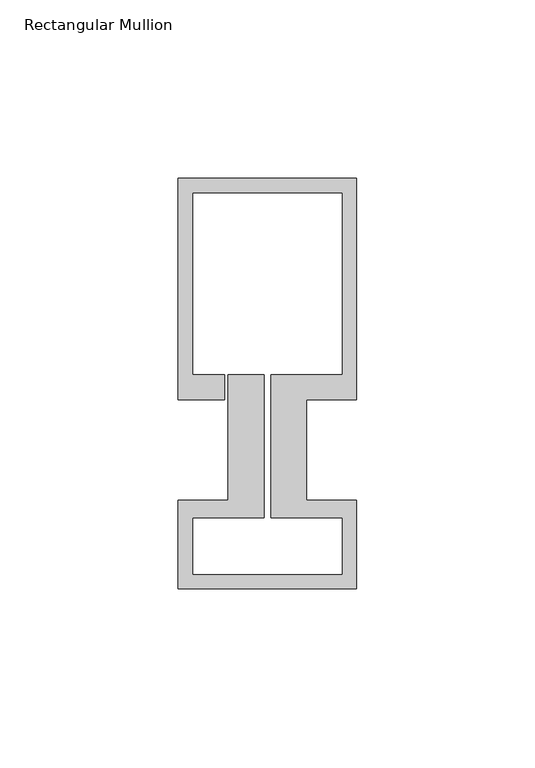
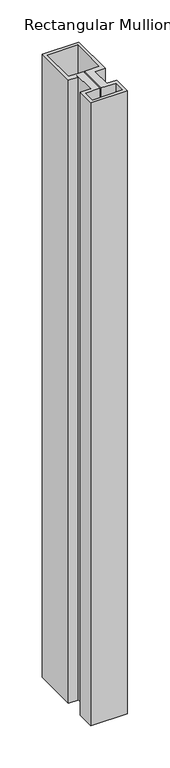
"""IFC4 building model written with IfcOpenShell, lengths in millimetres: member geometry, Rectangular Mullion : Schueco_FWS-50-HI_Tran_CovCap-20mm_Tran-55mm."""

from ifc_helpers import new_model, si_unit, frame, origin, place, context, project, spatial, polyline, outline, extrude, source, transform, mapped, element, save


def rectangular_mullion_16556d00(model_context):
    return source(origin(), model_context, "Body", "SweptSolid", [
        extrude(outline(polyline([(0.0, 90.0), (0.0, 28.0), (-14.0, 28.0), (-14.0, -0.1), (0.0, -0.1), (0.0, -25.0), (-50.0, -25.0), (-50.0, -0.1), (-36.0, -0.1), (-36.0, 35.0), (-26.0, 35.0), (-26.0, -5.0), (-46.0, -5.0), (-46.0, -21.0), (-4.0, -21.0), (-4.0, -5.0), (-24.0, -5.0), (-24.0, 35.0), (-4.0, 35.0), (-4.0, 86.0), (-46.0, 86.0), (-46.0, 35.0), (-37.0, 35.0), (-37.0, 28.0), (-50.0, 28.0), (-50.0, 90.0), (0.0, 90.0)])), frame((0.0, 0.0, -900.0), z_axis=(0.0, 0.0, 1.0), x_axis=(1.0, 0.0, 0.0)), (0.0, 0.0, 1.0), 900.0),
    ])


if __name__ == "__main__":
    model = new_model("IFC4")
    model_context = context("Model", 3, world=origin())
    ifc_project = project(units=[si_unit("LENGTHUNIT", "METRE", prefix="MILLI")], contexts=[model_context])
    site = spatial("IfcSite", under=ifc_project)
    building = spatial("IfcBuilding", under=site)
    placement = place(None, origin())
    rectangular_mullion_shape = rectangular_mullion_16556d00(model_context)
    element("IfcMember", 1, ObjectType="Rectangular Mullion : Schueco_FWS-50-HI_Tran_CovCap-20mm_Tran-55mm", at=placement, inside=building, context=model_context, shape_type="MappedRepresentation", body=[
        mapped(rectangular_mullion_shape, transform((0.0, 0.0, 0.0), x_axis=(1.0, 0.0, 0.0), y_axis=(0.0, 1.0, 0.0), z_axis=(0.0, 0.0, 1.0))),
    ])
    save(model, "model.ifc")

# Revit data of these elements
# Type "Rectangular Mullion : Schueco_FWS-50-HI_Tran_CovCap-20mm_Tran-55mm"
#   Model = "FWS 50.HI"
#   Manufacturer = "Schueco International KG"
#   Type Comments = "Transom"
#   Schueco thermal insulation standard = "Highly thermally insulated"
#   Burglar resistance = "RC 3"
#   Thermal insulation = "to 0.90 W/(m²K)"
#   built-in parameter 1007322 = 0.377297 (stored number, unit not read)
#   built-in parameter 1007321 = 0.0360892 (stored number, unit not read)
#   built-in parameter 1007320 = 0.0360892 (stored number, unit not read)
# Element 1 (IfcMember, "Rectangular Mullion : Schueco_FWS-50-HI_Tran_CovCap-20mm_Tran-55mm")
#   Materials on its faces: "Alu"
# Materials
#   "Alu": class "Glas", colour RGB 140 140 140, transparency 0
